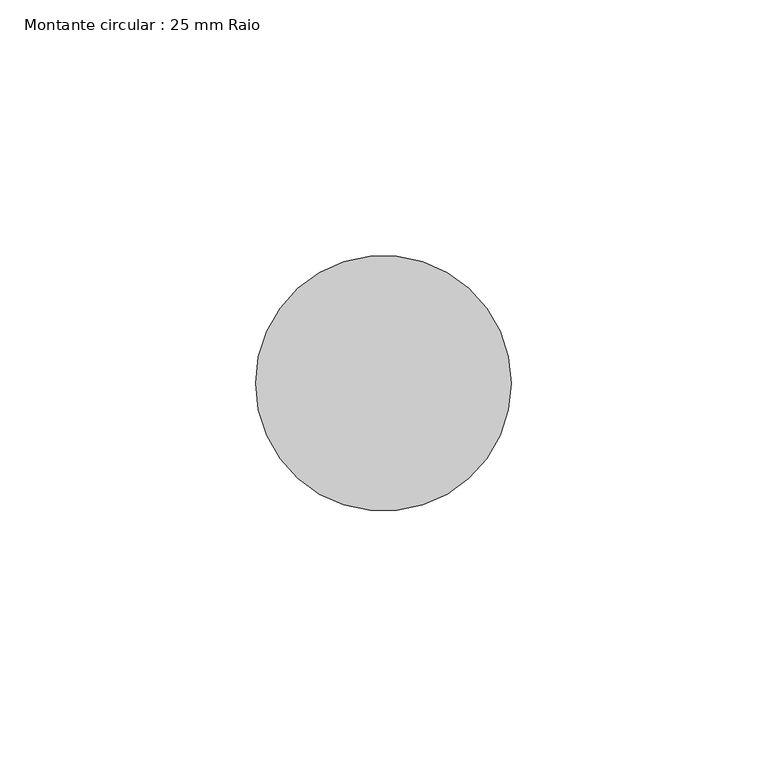
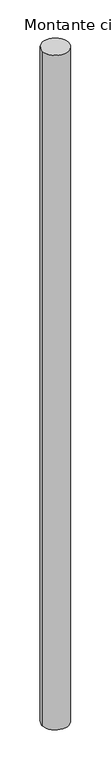
"""IFC4 building model written with IfcOpenShell, lengths in millimetres: member geometry, Montante circular : 25 mm Raio."""

from ifc_helpers import new_model, si_unit, point, frame, origin, origin_2d, place, context, project, spatial, circle_curve, trimmed, segment, composite_curve, outline, extrude, source, transform, mapped, element, save


def montante_circular_25_mm_raio_a3d7ebaf(model_context):
    return source(origin(), model_context, "Body", "SweptSolid", [
        extrude(outline(composite_curve([segment(trimmed(circle_curve(origin_2d(), 25.0), [point((25.0, 0.0))], [point((-25.0, 0.0))], False, "CARTESIAN"), True, "CONTINUOUS"), segment(trimmed(circle_curve(origin_2d(), 25.0), [point((-25.0, 0.0))], [point((25.0, 0.0))], False, "CARTESIAN"), True, "CONTINUOUS")], self_intersect=False)), frame((0.0, 0.0, -1357.623608), z_axis=(0.0, 0.0, 1.0), x_axis=(1.0, 0.0, 0.0)), (0.0, 0.0, 1.0), 1357.623608),
    ])


if __name__ == "__main__":
    model = new_model("IFC4")
    model_context = context("Model", 3, world=origin())
    ifc_project = project(units=[si_unit("LENGTHUNIT", "METRE", prefix="MILLI")], contexts=[model_context])
    site = spatial("IfcSite", under=ifc_project)
    building = spatial("IfcBuilding", under=site)
    placement = place(None, origin())
    montante_circular_25_mm_raio_shape = montante_circular_25_mm_raio_a3d7ebaf(model_context)
    element("IfcMember", 1, ObjectType="Montante circular : 25 mm Raio", at=placement, inside=building, context=model_context, shape_type="MappedRepresentation", body=[
        mapped(montante_circular_25_mm_raio_shape, transform((0.0, 0.0, 0.0), x_axis=(1.0, 0.0, 0.0), y_axis=(0.0, 1.0, 0.0), z_axis=(0.0, 0.0, 1.0))),
    ])
    save(model, "model.ifc")

# Revit data of these elements
# Type "Montante circular : 25 mm Raio"
#   built-in parameter 1007350 = 0.082021 (stored number, unit not read)
# Element 1 (IfcMember, "Montante circular : 25 mm Raio")
#   Materials on its faces: "Alumín."
# Materials
#   "Alumín.": class "Metal", colour RGB 247 247 247, transparency 0, Description = "Alumín. 6061", Cost = 0
